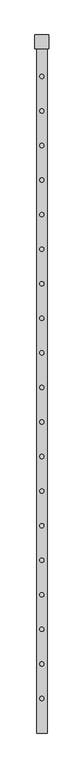
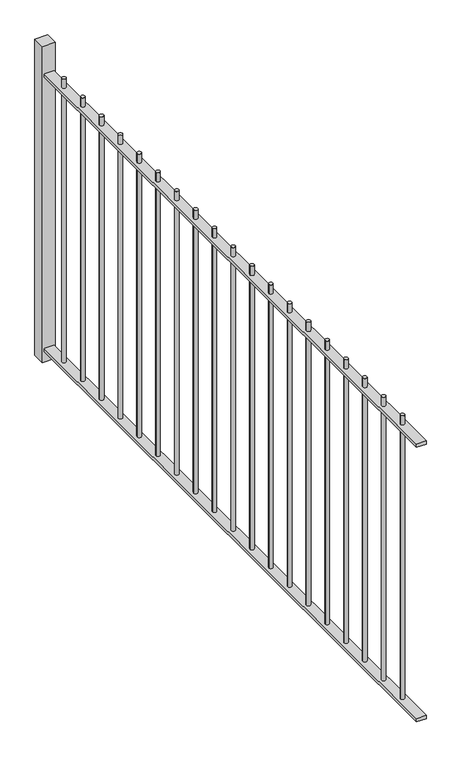
"""IFC4 building model written with IfcOpenShell, lengths in millimetres: railing geometry."""

from ifc_helpers import new_model, si_unit, point, frame, frame_2d, origin, place, context, project, spatial, polyline, circle_curve, trimmed, segment, composite_curve, outline, extrude, source, transform, mapped, element, save


def railing_98671243(model_context):
    return source(origin(), model_context, "Body", "SweptSolid", [
        extrude(outline(polyline([(-6549.419961, -4731.1119119), (-6489.419961, -4731.1119119), (-6489.419961, -8731.1119119), (-6549.419961, -8731.1119119), (-6549.419961, -4731.1119119)])), frame((0.0, 0.0, -30.0), z_axis=(0.0, 0.0, 1.0), x_axis=(1.0, 0.0, 0.0)), (0.0, 0.0, 1.0), 20.0),
        extrude(outline(polyline([(-6549.419961, -4731.1119119), (-6489.419961, -4731.1119119), (-6489.419961, -8731.1119119), (-6549.419961, -8731.1119119), (-6549.419961, -4731.1119119)])), frame((0.0, 0.0, 1750.0), z_axis=(0.0, 0.0, 1.0), x_axis=(1.0, 0.0, 0.0)), (0.0, 0.0, 1.0), 20.0),
        extrude(outline(composite_curve([segment(trimmed(circle_curve(frame_2d((-6519.419961, -8531.1119119)), 12.5), [point((-6531.919961, -8531.1119119))], [point((-6506.919961, -8531.1119119))], False, "CARTESIAN"), True, "CONTINUOUS"), segment(trimmed(circle_curve(frame_2d((-6519.419961, -8531.1119119)), 12.5), [point((-6506.919961, -8531.1119119))], [point((-6531.919961, -8531.1119119))], False, "CARTESIAN"), True, "CONTINUOUS")], self_intersect=False)), frame((0.0, 0.0, -10.0), z_axis=(0.0, 0.0, 1.0), x_axis=(1.0, 0.0, 0.0)), (0.0, 0.0, 1.0), 1840.0),
        extrude(outline(composite_curve([segment(trimmed(circle_curve(frame_2d((-6519.419961, -8331.1119119)), 12.5), [point((-6531.919961, -8331.1119119))], [point((-6506.919961, -8331.1119119))], False, "CARTESIAN"), True, "CONTINUOUS"), segment(trimmed(circle_curve(frame_2d((-6519.419961, -8331.1119119)), 12.5), [point((-6506.919961, -8331.1119119))], [point((-6531.919961, -8331.1119119))], False, "CARTESIAN"), True, "CONTINUOUS")], self_intersect=False)), frame((0.0, 0.0, -10.0), z_axis=(0.0, 0.0, 1.0), x_axis=(1.0, 0.0, 0.0)), (0.0, 0.0, 1.0), 1840.0),
        extrude(outline(composite_curve([segment(trimmed(circle_curve(frame_2d((-6519.419961, -8131.1119119)), 12.5), [point((-6531.919961, -8131.1119119))], [point((-6506.919961, -8131.1119119))], False, "CARTESIAN"), True, "CONTINUOUS"), segment(trimmed(circle_curve(frame_2d((-6519.419961, -8131.1119119)), 12.5), [point((-6506.919961, -8131.1119119))], [point((-6531.919961, -8131.1119119))], False, "CARTESIAN"), True, "CONTINUOUS")], self_intersect=False)), frame((0.0, 0.0, -10.0), z_axis=(0.0, 0.0, 1.0), x_axis=(1.0, 0.0, 0.0)), (0.0, 0.0, 1.0), 1840.0),
        extrude(outline(composite_curve([segment(trimmed(circle_curve(frame_2d((-6519.419961, -7931.1119119)), 12.5), [point((-6531.919961, -7931.1119119))], [point((-6506.919961, -7931.1119119))], False, "CARTESIAN"), True, "CONTINUOUS"), segment(trimmed(circle_curve(frame_2d((-6519.419961, -7931.1119119)), 12.5), [point((-6506.919961, -7931.1119119))], [point((-6531.919961, -7931.1119119))], False, "CARTESIAN"), True, "CONTINUOUS")], self_intersect=False)), frame((0.0, 0.0, -10.0), z_axis=(0.0, 0.0, 1.0), x_axis=(1.0, 0.0, 0.0)), (0.0, 0.0, 1.0), 1840.0),
        extrude(outline(composite_curve([segment(trimmed(circle_curve(frame_2d((-6519.419961, -7731.1119119)), 12.5), [point((-6531.919961, -7731.1119119))], [point((-6506.919961, -7731.1119119))], False, "CARTESIAN"), True, "CONTINUOUS"), segment(trimmed(circle_curve(frame_2d((-6519.419961, -7731.1119119)), 12.5), [point((-6506.919961, -7731.1119119))], [point((-6531.919961, -7731.1119119))], False, "CARTESIAN"), True, "CONTINUOUS")], self_intersect=False)), frame((0.0, 0.0, -10.0), z_axis=(0.0, 0.0, 1.0), x_axis=(1.0, 0.0, 0.0)), (0.0, 0.0, 1.0), 1840.0),
        extrude(outline(composite_curve([segment(trimmed(circle_curve(frame_2d((-6519.419961, -7531.1119119)), 12.5), [point((-6531.919961, -7531.1119119))], [point((-6506.919961, -7531.1119119))], False, "CARTESIAN"), True, "CONTINUOUS"), segment(trimmed(circle_curve(frame_2d((-6519.419961, -7531.1119119)), 12.5), [point((-6506.919961, -7531.1119119))], [point((-6531.919961, -7531.1119119))], False, "CARTESIAN"), True, "CONTINUOUS")], self_intersect=False)), frame((0.0, 0.0, -10.0), z_axis=(0.0, 0.0, 1.0), x_axis=(1.0, 0.0, 0.0)), (0.0, 0.0, 1.0), 1840.0),
        extrude(outline(composite_curve([segment(trimmed(circle_curve(frame_2d((-6519.419961, -7331.1119119)), 12.5), [point((-6531.919961, -7331.1119119))], [point((-6506.919961, -7331.1119119))], False, "CARTESIAN"), True, "CONTINUOUS"), segment(trimmed(circle_curve(frame_2d((-6519.419961, -7331.1119119)), 12.5), [point((-6506.919961, -7331.1119119))], [point((-6531.919961, -7331.1119119))], False, "CARTESIAN"), True, "CONTINUOUS")], self_intersect=False)), frame((0.0, 0.0, -10.0), z_axis=(0.0, 0.0, 1.0), x_axis=(1.0, 0.0, 0.0)), (0.0, 0.0, 1.0), 1840.0),
        extrude(outline(composite_curve([segment(trimmed(circle_curve(frame_2d((-6519.419961, -7131.1119119)), 12.5), [point((-6531.919961, -7131.1119119))], [point((-6506.919961, -7131.1119119))], False, "CARTESIAN"), True, "CONTINUOUS"), segment(trimmed(circle_curve(frame_2d((-6519.419961, -7131.1119119)), 12.5), [point((-6506.919961, -7131.1119119))], [point((-6531.919961, -7131.1119119))], False, "CARTESIAN"), True, "CONTINUOUS")], self_intersect=False)), frame((0.0, 0.0, -10.0), z_axis=(0.0, 0.0, 1.0), x_axis=(1.0, 0.0, 0.0)), (0.0, 0.0, 1.0), 1840.0),
        extrude(outline(composite_curve([segment(trimmed(circle_curve(frame_2d((-6519.419961, -6931.1119119)), 12.5), [point((-6531.919961, -6931.1119119))], [point((-6506.919961, -6931.1119119))], False, "CARTESIAN"), True, "CONTINUOUS"), segment(trimmed(circle_curve(frame_2d((-6519.419961, -6931.1119119)), 12.5), [point((-6506.919961, -6931.1119119))], [point((-6531.919961, -6931.1119119))], False, "CARTESIAN"), True, "CONTINUOUS")], self_intersect=False)), frame((0.0, 0.0, -10.0), z_axis=(0.0, 0.0, 1.0), x_axis=(1.0, 0.0, 0.0)), (0.0, 0.0, 1.0), 1840.0),
        extrude(outline(composite_curve([segment(trimmed(circle_curve(frame_2d((-6519.419961, -6731.1119119)), 12.5), [point((-6531.919961, -6731.1119119))], [point((-6506.919961, -6731.1119119))], False, "CARTESIAN"), True, "CONTINUOUS"), segment(trimmed(circle_curve(frame_2d((-6519.419961, -6731.1119119)), 12.5), [point((-6506.919961, -6731.1119119))], [point((-6531.919961, -6731.1119119))], False, "CARTESIAN"), True, "CONTINUOUS")], self_intersect=False)), frame((0.0, 0.0, -10.0), z_axis=(0.0, 0.0, 1.0), x_axis=(1.0, 0.0, 0.0)), (0.0, 0.0, 1.0), 1840.0),
        extrude(outline(composite_curve([segment(trimmed(circle_curve(frame_2d((-6519.419961, -6531.1119119)), 12.5), [point((-6531.919961, -6531.1119119))], [point((-6506.919961, -6531.1119119))], False, "CARTESIAN"), True, "CONTINUOUS"), segment(trimmed(circle_curve(frame_2d((-6519.419961, -6531.1119119)), 12.5), [point((-6506.919961, -6531.1119119))], [point((-6531.919961, -6531.1119119))], False, "CARTESIAN"), True, "CONTINUOUS")], self_intersect=False)), frame((0.0, 0.0, -10.0), z_axis=(0.0, 0.0, 1.0), x_axis=(1.0, 0.0, 0.0)), (0.0, 0.0, 1.0), 1840.0),
        extrude(outline(composite_curve([segment(trimmed(circle_curve(frame_2d((-6519.419961, -6331.1119119)), 12.5), [point((-6531.919961, -6331.1119119))], [point((-6506.919961, -6331.1119119))], False, "CARTESIAN"), True, "CONTINUOUS"), segment(trimmed(circle_curve(frame_2d((-6519.419961, -6331.1119119)), 12.5), [point((-6506.919961, -6331.1119119))], [point((-6531.919961, -6331.1119119))], False, "CARTESIAN"), True, "CONTINUOUS")], self_intersect=False)), frame((0.0, 0.0, -10.0), z_axis=(0.0, 0.0, 1.0), x_axis=(1.0, 0.0, 0.0)), (0.0, 0.0, 1.0), 1840.0),
        extrude(outline(composite_curve([segment(trimmed(circle_curve(frame_2d((-6519.419961, -6131.1119119)), 12.5), [point((-6531.919961, -6131.1119119))], [point((-6506.919961, -6131.1119119))], False, "CARTESIAN"), True, "CONTINUOUS"), segment(trimmed(circle_curve(frame_2d((-6519.419961, -6131.1119119)), 12.5), [point((-6506.919961, -6131.1119119))], [point((-6531.919961, -6131.1119119))], False, "CARTESIAN"), True, "CONTINUOUS")], self_intersect=False)), frame((0.0, 0.0, -10.0), z_axis=(0.0, 0.0, 1.0), x_axis=(1.0, 0.0, 0.0)), (0.0, 0.0, 1.0), 1840.0),
        extrude(outline(composite_curve([segment(trimmed(circle_curve(frame_2d((-6519.419961, -5931.1119119)), 12.5), [point((-6531.919961, -5931.1119119))], [point((-6506.919961, -5931.1119119))], False, "CARTESIAN"), True, "CONTINUOUS"), segment(trimmed(circle_curve(frame_2d((-6519.419961, -5931.1119119)), 12.5), [point((-6506.919961, -5931.1119119))], [point((-6531.919961, -5931.1119119))], False, "CARTESIAN"), True, "CONTINUOUS")], self_intersect=False)), frame((0.0, 0.0, -10.0), z_axis=(0.0, 0.0, 1.0), x_axis=(1.0, 0.0, 0.0)), (0.0, 0.0, 1.0), 1840.0),
        extrude(outline(composite_curve([segment(trimmed(circle_curve(frame_2d((-6519.419961, -5731.1119119)), 12.5), [point((-6531.919961, -5731.1119119))], [point((-6506.919961, -5731.1119119))], False, "CARTESIAN"), True, "CONTINUOUS"), segment(trimmed(circle_curve(frame_2d((-6519.419961, -5731.1119119)), 12.5), [point((-6506.919961, -5731.1119119))], [point((-6531.919961, -5731.1119119))], False, "CARTESIAN"), True, "CONTINUOUS")], self_intersect=False)), frame((0.0, 0.0, -10.0), z_axis=(0.0, 0.0, 1.0), x_axis=(1.0, 0.0, 0.0)), (0.0, 0.0, 1.0), 1840.0),
        extrude(outline(composite_curve([segment(trimmed(circle_curve(frame_2d((-6519.419961, -5531.1119119)), 12.5), [point((-6531.919961, -5531.1119119))], [point((-6506.919961, -5531.1119119))], False, "CARTESIAN"), True, "CONTINUOUS"), segment(trimmed(circle_curve(frame_2d((-6519.419961, -5531.1119119)), 12.5), [point((-6506.919961, -5531.1119119))], [point((-6531.919961, -5531.1119119))], False, "CARTESIAN"), True, "CONTINUOUS")], self_intersect=False)), frame((0.0, 0.0, -10.0), z_axis=(0.0, 0.0, 1.0), x_axis=(1.0, 0.0, 0.0)), (0.0, 0.0, 1.0), 1840.0),
        extrude(outline(composite_curve([segment(trimmed(circle_curve(frame_2d((-6519.419961, -5331.1119119)), 12.5), [point((-6531.919961, -5331.1119119))], [point((-6506.919961, -5331.1119119))], False, "CARTESIAN"), True, "CONTINUOUS"), segment(trimmed(circle_curve(frame_2d((-6519.419961, -5331.1119119)), 12.5), [point((-6506.919961, -5331.1119119))], [point((-6531.919961, -5331.1119119))], False, "CARTESIAN"), True, "CONTINUOUS")], self_intersect=False)), frame((0.0, 0.0, -10.0), z_axis=(0.0, 0.0, 1.0), x_axis=(1.0, 0.0, 0.0)), (0.0, 0.0, 1.0), 1840.0),
        extrude(outline(composite_curve([segment(trimmed(circle_curve(frame_2d((-6519.419961, -5131.1119119)), 12.5), [point((-6531.919961, -5131.1119119))], [point((-6506.919961, -5131.1119119))], False, "CARTESIAN"), True, "CONTINUOUS"), segment(trimmed(circle_curve(frame_2d((-6519.419961, -5131.1119119)), 12.5), [point((-6506.919961, -5131.1119119))], [point((-6531.919961, -5131.1119119))], False, "CARTESIAN"), True, "CONTINUOUS")], self_intersect=False)), frame((0.0, 0.0, -10.0), z_axis=(0.0, 0.0, 1.0), x_axis=(1.0, 0.0, 0.0)), (0.0, 0.0, 1.0), 1840.0),
        extrude(outline(composite_curve([segment(trimmed(circle_curve(frame_2d((-6519.419961, -4931.1119119)), 12.5), [point((-6531.919961, -4931.1119119))], [point((-6506.919961, -4931.1119119))], False, "CARTESIAN"), True, "CONTINUOUS"), segment(trimmed(circle_curve(frame_2d((-6519.419961, -4931.1119119)), 12.5), [point((-6506.919961, -4931.1119119))], [point((-6531.919961, -4931.1119119))], False, "CARTESIAN"), True, "CONTINUOUS")], self_intersect=False)), frame((0.0, 0.0, -10.0), z_axis=(0.0, 0.0, 1.0), x_axis=(1.0, 0.0, 0.0)), (0.0, 0.0, 1.0), 1840.0),
        extrude(outline(polyline([(-6479.419961, -4691.1119119), (-6479.419961, -4771.1119119), (-6559.419961, -4771.1119119), (-6559.419961, -4691.1119119), (-6479.419961, -4691.1119119)])), frame((0.0, 0.0, -100.0), z_axis=(0.0, 0.0, 1.0), x_axis=(1.0, 0.0, 0.0)), (0.0, 0.0, 1.0), 2050.0),
    ])


if __name__ == "__main__":
    model = new_model("IFC4")
    model_context = context("Model", 3, world=origin())
    ifc_project = project(units=[si_unit("LENGTHUNIT", "METRE", prefix="MILLI")], contexts=[model_context])
    site = spatial("IfcSite", under=ifc_project)
    building = spatial("IfcBuilding", under=site)
    placement = place(None, origin())
    railing_shape = railing_98671243(model_context)
    element("IfcRailing", 1, at=placement, inside=building, context=model_context, shape_type="MappedRepresentation", body=[
        mapped(railing_shape, transform((0.0, 0.0, 0.0), x_axis=(1.0, 0.0, 0.0), y_axis=(0.0, 1.0, 0.0), z_axis=(0.0, 0.0, 1.0))),
    ])
    save(model, "model.ifc")

# Revit data of these elements
# Element 1 (IfcRailing)
#   Materials on its faces: "NLRS_h2_staal_generiek zwart_gen_rsf", "NLRS_h2_staal_gen_rsf"
# Materials
#   "NLRS_h2_staal_generiek zwart_gen_rsf": class "Metal", colour RGB 189 187 185, transparency 0, Manufacturer = "RevitGG", URL = "www.revitgg.nl", Description = "Staal, generiek materiaal", Cost = 0
#   "NLRS_h2_staal_gen_rsf": class "H - Metaal", colour RGB 189 187 185, transparency 0, Keynote = "h2", Model = "generiek", Manufacturer = "Revit Standards Foundation", URL = "www.revitstandards.org", Description = "staal", Cost = 0
